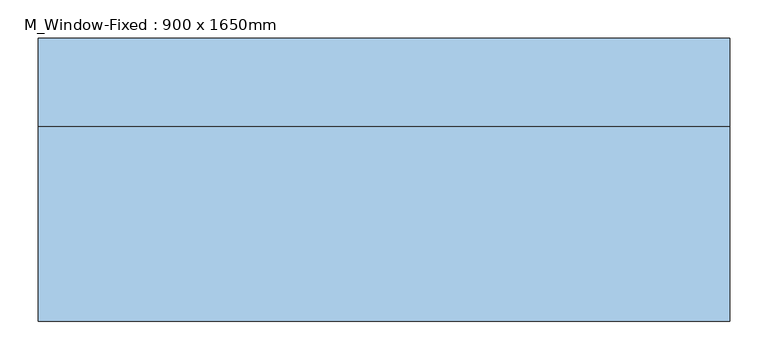
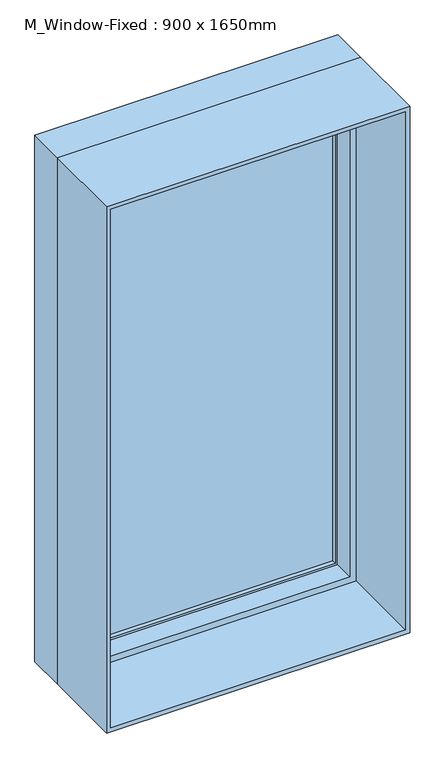
"""IFC4 building model written with IfcOpenShell, lengths in millimetres: window geometry, M_Window-Fixed : 900 x 1650mm."""

import ifcopenshell
import ifcopenshell.guid

model = None  # the IFC model being written
_history = None  # IfcOwnerHistory: only IFC2X3 demands one
_inside = {}  # id of a spatial element -> (the spatial element, [elements in it])
_under = {}  # id of a project, library or spatial element -> (it, [spatial elements below it])
_declared = {}  # id of a project -> (the project, [libraries it declares])
_typed = {}  # id of a type object -> (the type object, [elements of that type])
_made_of = {}  # id of a material, layer set ... -> (it, [elements and type objects made of it])


def new_model(schema):
    """Start an empty IFC model of exactly this schema.

    Asked for "IFC4X3", IfcOpenShell would pick the latest addendum, in which some entities
    have other attributes; the version numbers below select the first issue.
    IFC2X3 requires an IfcOwnerHistory on every rooted entity: one is made here for all.
    """
    global model, _history
    if schema == "IFC4X3":
        model = ifcopenshell.file(schema_version=(4, 3, 0, 0))
    else:
        model = ifcopenshell.file(schema=schema)
    _inside.clear()
    _under.clear()
    _declared.clear()
    _typed.clear()
    _made_of.clear()
    _history = None
    if model.schema == "IFC2X3":
        org = make("IfcOrganization", Name="unknown")
        user = make(
            "IfcPersonAndOrganization",
            ThePerson=make("IfcPerson", FamilyName="unknown"),
            TheOrganization=org,
        )
        app = make(
            "IfcApplication",
            ApplicationDeveloper=org,
            Version="unknown",
            ApplicationFullName="unknown",
            ApplicationIdentifier="unknown",
        )
        _history = make(
            "IfcOwnerHistory",
            OwningUser=user,
            OwningApplication=app,
            ChangeAction="ADDED",
            CreationDate=0,
        )
    return model


def make(cls, **values):
    """One entity of the class cls with the attributes given. An attribute that is None is left unset."""
    return model.create_entity(
        cls, **{name: value for name, value in values.items() if value is not None}
    )


def rooted(cls, **values):
    """An entity with a GlobalId (a new one), such as an element, a storey or a relation."""
    return make(cls, GlobalId=ifcopenshell.guid.new(), OwnerHistory=_history, **values)


def si_unit(unit_type, name, prefix=None):
    """IfcSIUnit, for example si_unit("LENGTHUNIT", "METRE", prefix="MILLI")."""
    return make("IfcSIUnit", UnitType=unit_type, Prefix=prefix, Name=name)


def assignment(units):
    """IfcUnitAssignment: the units of a project."""
    return None if units is None else make("IfcUnitAssignment", Units=units)


def point(xyz):
    """IfcCartesianPoint."""
    return None if xyz is None else make("IfcCartesianPoint", Coordinates=xyz)


def direction(xyz):
    """IfcDirection."""
    return None if xyz is None else make("IfcDirection", DirectionRatios=xyz)


def frame(location, z_axis=None, x_axis=None):
    """IfcAxis2Placement3D, a coordinate frame: its origin and axes. An axis left out is left unset."""
    return make(
        "IfcAxis2Placement3D",
        Location=point(location),
        Axis=direction(z_axis),
        RefDirection=direction(x_axis),
    )


def origin():
    """The frame at (0, 0, 0) with its axes left unset."""
    return frame((0.0, 0.0, 0.0))


def place(relative_to, where):
    """IfcLocalPlacement: puts the frame where relative to a parent placement (None: the world)."""
    return make(
        "IfcLocalPlacement", PlacementRelTo=relative_to, RelativePlacement=where
    )


def context(
    kind, dimensions, precision=None, world=None, true_north=None, identifier=None
):
    """IfcGeometricRepresentationContext, for example the 3D "Model" context."""
    return make(
        "IfcGeometricRepresentationContext",
        ContextIdentifier=identifier,
        ContextType=kind,
        CoordinateSpaceDimension=dimensions,
        Precision=precision,
        WorldCoordinateSystem=world,
        TrueNorth=true_north,
    )


def project(units=None, contexts=None):
    """IfcProject with its units and contexts."""
    return rooted(
        "IfcProject",
        Name="project",
        RepresentationContexts=contexts,
        UnitsInContext=assignment(units),
    )


def spatial(cls, under=None, at=None, **own):
    """A site, building, storey or space (cls), placed at a placement, below another one or the project."""
    s = rooted(cls, ObjectPlacement=at, **own)
    if under is not None:
        _under.setdefault(under.id(), (under, []))[1].append(s)
    return s


def polyline(points):
    """IfcPolyline through the points."""
    return make("IfcPolyline", Points=[point(p) for p in points])


def outline(outer, holes=None, kind="AREA"):
    """IfcArbitraryClosedProfileDef: a profile drawn as a closed curve; with holes, ...WithVoids."""
    if holes is None:
        return make("IfcArbitraryClosedProfileDef", ProfileType=kind, OuterCurve=outer)
    return make(
        "IfcArbitraryProfileDefWithVoids",
        ProfileType=kind,
        OuterCurve=outer,
        InnerCurves=holes,
    )


def extrude(swept, where, along, depth):
    """IfcExtrudedAreaSolid: the profile swept, set in the frame where, extruded along a direction by depth."""
    return make(
        "IfcExtrudedAreaSolid",
        SweptArea=swept,
        Position=where,
        ExtrudedDirection=direction(along),
        Depth=depth,
    )


def faces_of(points, faces, orient=None, outer=None):
    """IfcFace entities. A face is a list of loops; a loop is a list of indices into points, from 0.

    orient and outer hold one flag for each loop. By default every Orientation is true, the
    first loop of a face is its IfcFaceOuterBound and the others are IfcFaceBound.
    """
    made = []
    for i, loops in enumerate(faces):
        bounds = []
        for j, loop in enumerate(loops):
            is_outer = j == 0 if outer is None else outer[i][j]
            bounds.append(
                make(
                    "IfcFaceOuterBound" if is_outer else "IfcFaceBound",
                    Bound=make("IfcPolyLoop", Polygon=[points[k] for k in loop]),
                    Orientation=True if orient is None else orient[i][j],
                )
            )
        made.append(make("IfcFace", Bounds=bounds))
    return made


def faceted_brep(points, faces, orient=None, outer=None, voids=None):
    """IfcFacetedBrep: a solid bounded by flat faces; with voids (closed shells), ...WithVoids."""
    shared = [point(p) for p in points]
    hull = make("IfcClosedShell", CfsFaces=faces_of(shared, faces, orient, outer))
    if voids is None:
        return make("IfcFacetedBrep", Outer=hull)
    return make(
        "IfcFacetedBrepWithVoids",
        Outer=hull,
        Voids=[
            make(cls, CfsFaces=faces_of(shared, fs, o, b)) for cls, fs, o, b in voids
        ],
    )


def shape(context_of_items, identifier, shape_type, items):
    """IfcShapeRepresentation: the items that make up one representation, for example the "Body"."""
    return make(
        "IfcShapeRepresentation",
        ContextOfItems=context_of_items,
        RepresentationIdentifier=identifier,
        RepresentationType=shape_type,
        Items=items,
    )


def source(mapping_origin, context_of_items, identifier, shape_type, items):
    """IfcRepresentationMap: a shape defined once, which mapped items show again and again."""
    return make(
        "IfcRepresentationMap",
        MappingOrigin=mapping_origin,
        MappedRepresentation=shape(context_of_items, identifier, shape_type, items),
    )


def transform(
    local_origin,
    x_axis=None,
    y_axis=None,
    z_axis=None,
    scale=None,
    scale2=None,
    scale3=None,
    uniform=True,
):
    """IfcCartesianTransformationOperator3D, or its non-uniform kind. x_axis, y_axis, z_axis: its Axis1, 2, 3."""
    if uniform:
        return make(
            "IfcCartesianTransformationOperator3D",
            Axis1=direction(x_axis),
            Axis2=direction(y_axis),
            LocalOrigin=point(local_origin),
            Scale=scale,
            Axis3=direction(z_axis),
        )
    return make(
        "IfcCartesianTransformationOperator3DnonUniform",
        Axis1=direction(x_axis),
        Axis2=direction(y_axis),
        LocalOrigin=point(local_origin),
        Scale=scale,
        Axis3=direction(z_axis),
        Scale2=scale2,
        Scale3=scale3,
    )


def mapped(mapping_source, mapping_target):
    """IfcMappedItem: shows the shape of a source again, moved by a transform."""
    return make(
        "IfcMappedItem", MappingSource=mapping_source, MappingTarget=mapping_target
    )


def made_of(thing, what):
    """Note that an element or type object is made of a material, layer set ...; save() writes the relation."""
    if what is not None:
        _made_of.setdefault(what.id(), (what, []))[1].append(thing)
    return thing


def element(
    cls,
    number,
    at=None,
    inside=None,
    cuts=None,
    type_object=None,
    material=None,
    context=None,
    identifier="Body",
    shape_type=None,
    held_by="IfcProductDefinitionShape",
    body=None,
    shapes=None,
    **own,
):
    """One element of the class cls, such as IfcWall. Its Tag is "e" and its number.

    at: its placement. inside: the storey or other place that contains it. cuts: it is an
    opening in that element (IfcRelVoidsElement). A single representation is given by context,
    identifier, shape_type and body (its items); several are given by shapes. held_by: the class
    of the entity that holds the representations. save() writes the other relations.
    """
    e = rooted(cls, Tag="e%d" % number, ObjectPlacement=at, **own)
    if body is not None:
        shapes = [shape(context, identifier, shape_type, body)]
    if shapes is not None:
        e.Representation = make(held_by, Representations=shapes)
    if inside is not None:
        _inside.setdefault(inside.id(), (inside, []))[1].append(e)
    if cuts is not None:
        rooted(
            "IfcRelVoidsElement", RelatingBuildingElement=cuts, RelatedOpeningElement=e
        )
    if type_object is not None:
        _typed.setdefault(type_object.id(), (type_object, []))[1].append(e)
    return made_of(e, material)


def aggregate(whole, parts):
    """IfcRelAggregates: a whole, such as a stair, and the parts it consists of."""
    return rooted("IfcRelAggregates", RelatingObject=whole, RelatedObjects=parts)


def save(model, path):
    """Write the relations noted so far, then the file.

    IfcRelAggregates (storeys below a building ...), IfcRelContainedInSpatialStructure (elements
    in a storey), IfcRelDefinesByType, IfcRelAssociatesMaterial and IfcRelDeclares: one each for
    every whole, place, type object, material and project.
    """
    for whole, parts in _under.values():
        aggregate(whole, parts)
    for where, things in _inside.values():
        rooted(
            "IfcRelContainedInSpatialStructure",
            RelatedElements=things,
            RelatingStructure=where,
        )
    for kind, things in _typed.values():
        rooted("IfcRelDefinesByType", RelatedObjects=things, RelatingType=kind)
    for what, things in _made_of.values():
        rooted("IfcRelAssociatesMaterial", RelatedObjects=things, RelatingMaterial=what)
    for by, libraries in _declared.values():
        rooted("IfcRelDeclares", RelatingContext=by, RelatedDefinitions=libraries)
    model.write(path)


def m_window_fixed_900_x_1650mm_30845197(model_context):
    return source(origin(), model_context, "Body", "SolidModel", [
        faceted_brep([(450.0, 79.25, 2550.0), (450.0, 193.55, 2550.0), (-450.0, 193.55, 2550.0), (-450.0, 79.25, 2550.0), (-450.0, 193.55, 900.0), (-450.0, 79.25, 900.0), (450.0, 193.55, 900.0), (450.0, 79.25, 900.0), (418.25, 79.25, 2518.25), (418.25, 79.25, 931.75), (-418.25, 79.25, 931.75), (-418.25, 79.25, 2518.25), (-437.3, 193.55, 2537.3), (-437.3, 193.55, 912.7), (437.3, 193.55, 912.7), (437.3, 193.55, 2537.3), (418.25, 142.75, 2518.25), (-418.25, 142.75, 2518.25), (437.3, 142.75, 2537.3), (-437.3, 142.75, 2537.3), (-418.25, 142.75, 931.75), (-437.3, 142.75, 912.7), (418.25, 142.75, 931.75), (437.3, 142.75, 912.7)], [[[0, 1, 2, 3]], [[3, 2, 4, 5]], [[5, 4, 6, 7]], [[3, 5, 7, 0], [8, 9, 10, 11]], [[7, 6, 1, 0]], [[1, 6, 4, 2], [12, 13, 14, 15]], [[16, 8, 11, 17]], [[15, 18, 19, 12]], [[17, 11, 10, 20]], [[12, 19, 21, 13]], [[20, 10, 9, 22]], [[13, 21, 23, 14]], [[22, 9, 8, 16]], [[18, 23, 21, 19], [17, 20, 22, 16]], [[14, 23, 18, 15]]]),
        extrude(outline(polyline([(2550.0, -450.0), (900.0, -450.0), (900.0, 450.0), (2550.0, 450.0), (2550.0, -450.0)]), holes=[polyline([(2537.3, 437.3), (912.7, 437.3), (912.7, -437.3), (2537.3, -437.3), (2537.3, 437.3)])]), frame((0.0, -174.5, 0.0), z_axis=(0.0, 1.0, 0.0), x_axis=(0.0, 0.0, 1.0)), (0.0, 0.0, 1.0), 253.75),
        extrude(outline(polyline([(912.7, 437.3), (2537.3, 437.3), (2537.3, -437.3), (912.7, -437.3), (912.7, 437.3)]), holes=[polyline([(938.1, -411.9), (2511.9, -411.9), (2511.9, 411.9), (938.1, 411.9), (938.1, -411.9)])]), frame((0.0, 142.75, 0.0), z_axis=(0.0, 1.0, 0.0), x_axis=(0.0, 0.0, 1.0)), (0.0, 0.0, 1.0), 44.45),
        extrude(outline(polyline([(411.9, 174.5), (411.9, 168.15), (-411.9, 168.15), (-411.9, 174.5), (411.9, 174.5)])), frame((0.0, 0.0, 938.1), z_axis=(0.0, 0.0, 1.0), x_axis=(1.0, 0.0, 0.0)), (0.0, 0.0, 1.0), 1573.8),
        extrude(outline(polyline([(-411.9, 155.45), (-411.9, 161.8), (411.9, 161.8), (411.9, 155.45), (-411.9, 155.45)])), frame((0.0, 0.0, 938.1), z_axis=(0.0, 0.0, 1.0), x_axis=(1.0, 0.0, 0.0)), (0.0, 0.0, 1.0), 1573.8),
    ])


if __name__ == "__main__":
    model = new_model("IFC4")
    model_context = context("Model", 3, world=origin())
    ifc_project = project(units=[si_unit("LENGTHUNIT", "METRE", prefix="MILLI")], contexts=[model_context])
    site = spatial("IfcSite", under=ifc_project)
    building = spatial("IfcBuilding", under=site)
    placement = place(None, origin())
    m_window_fixed_900_x_1650mm_shape = m_window_fixed_900_x_1650mm_30845197(model_context)
    element("IfcWindow", 1, ObjectType="M_Window-Fixed : 900 x 1650mm", at=placement, inside=building, context=model_context, shape_type="MappedRepresentation", body=[
        mapped(m_window_fixed_900_x_1650mm_shape, transform((0.0, 0.0, 0.0), x_axis=(1.0, 0.0, 0.0), y_axis=(0.0, 1.0, 0.0), z_axis=(0.0, 0.0, 1.0))),
    ])
    save(model, "model.ifc")

# Revit data of these elements
# Type "M_Window-Fixed : 900 x 1650mm"
#   Type Mark = "38"
#   Fire Rating = "0.5h"
#   Assembly Code = "B2020100"
#   Analytic Construction = "Double glazing - domestic"
#   Window Inset [instance default] = 0 mm
#   Wall Thickness [instance default] = 150 mm
#   Visual Light Transmittance = 0.81
#   Thermal Resistance (R) = 0.319569 (m²·K)/W
#   Solar Heat Gain Coefficient = 0.76
#   Rough Width = 915 mm
#   Rough Height = 1665 mm
#   Interior Wall Closure [instance default] = 54.75 mm
#   Height = 1650 mm
#   Heat Transfer Coefficient (U) = 3.12929 W/(m²·K)
#   Frame Extension [instance default] = 6.35 mm
#   Exterior Wall Closure [instance default] = 31.75 mm
#   Extension Jamb [instance default] = 54.75 mm
#   Default Sill Height = 900 mm
#   Width = 900 mm
#   Muntin Visibility = yes
#   Interior Trim Visibility [instance default] = yes
#   Exterior Trim Visibility [instance default] = yes
#   Extension Jamb Visibility [instance default] = yes
#   Muntin Pattern = M_Muntin Pattern_2x2 : M_Muntin Pattern_2x2
#   Interior Trim Material = Wood - Stained
#   Interior Trim = M_Trim-Window-Interior-Flat : Picture Frame
#   Interior Frame Material = Wood - Stained
#   Glass Panel Material = Glass
#   Exterior Trim Material = Clad - White
#   Exterior Trim = M_Trim-Window-Exterior-Flat : with Sill
#   Exterior Frame Material = Clad - White
#   Wall Closure = (empty or 0)
# Element 1 (IfcWindow, "M_Window-Fixed : 900 x 1650mm")
#   Wall Thickness = 349 mm
#   Extension Jamb = 253.75 mm
#   Materials on its faces: "Wood - Stained", "Glass", "Clad - White"
# Materials
#   "Wood - Stained": class "Wood", colour RGB 173 132 96, transparency 0, Cost = 0
#   "Glass": class "Glass", colour RGB 245 245 243, transparency 1, Description = "Soda Lime Glass", Cost = 0
#   "Clad - White": class "Wood", colour RGB 245 245 243, transparency 0, Cost = 0
